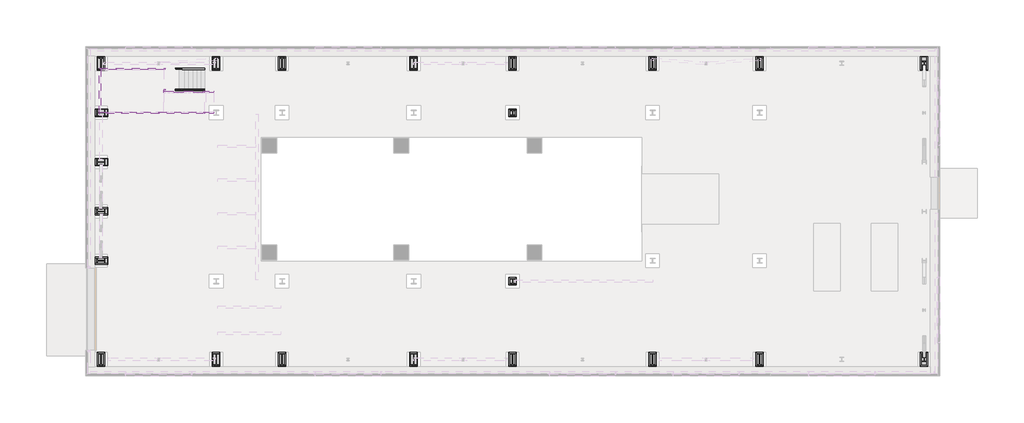
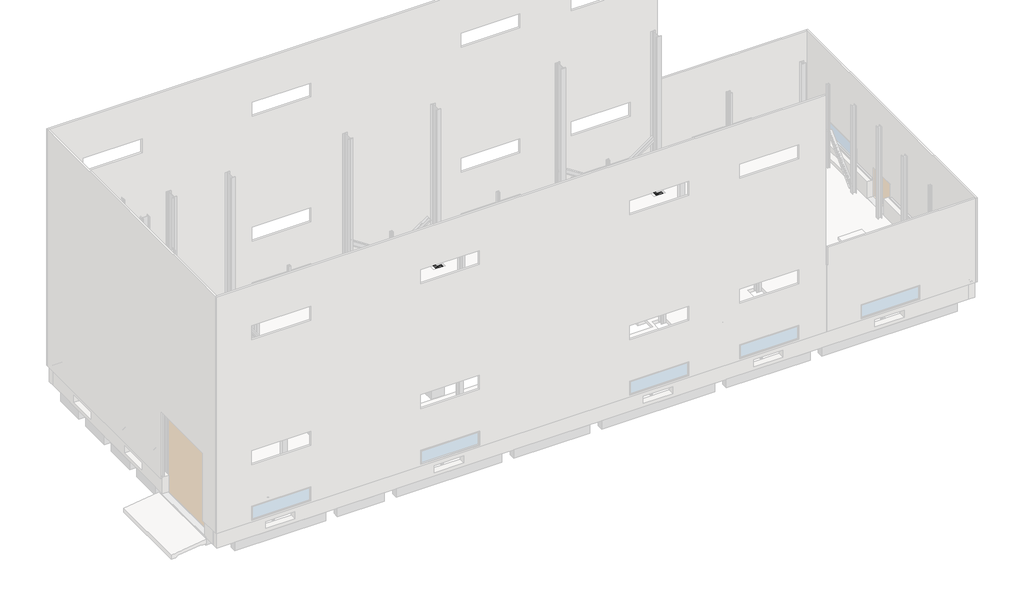
# One storey, part 4 of 4: 23 proxies, 10 members.
# Revit data of these elements (continued)
# Type "그라우트9 : 그라우트"
#   Description = ""
# Type "C-250X90"
#   Keynote = "ㄷ-250×90x9x13"
# Element 1 (IfcBuildingElementProxy, "그라우트 : 그라우트")
#   Phase Created = New Construction
# Element 2 (IfcBuildingElementProxy, "그라우트1 : 그라우트")
#   Phase Created = New Construction
# Element 3 (IfcBuildingElementProxy, "그라우트2 : 그라우트")
#   Phase Created = New Construction
# Element 4 (IfcBuildingElementProxy, "그라우트3 : 그라우트")
#   Phase Created = New Construction
# Element 5 (IfcBuildingElementProxy, "그라우트4 : 그라우트")
#   Phase Created = New Construction
# Element 6 (IfcBuildingElementProxy, "그라우트5 : 그라우트")
#   Phase Created = New Construction
# Element 7 (IfcBuildingElementProxy, "그라우트6 : 그라우트")
#   Phase Created = New Construction
# Element 8 (IfcBuildingElementProxy, "그라우트7 : 그라우트")
#   Phase Created = New Construction
# Element 9 (IfcBuildingElementProxy, "그라우트8 : 그라우트")
#   Phase Created = New Construction
# Element 10 (IfcBuildingElementProxy, "그라우트9 : 그라우트")
#   Phase Created = New Construction
# Element 11 (IfcBuildingElementProxy, "그라우트10 : 그라우트")
#   Phase Created = New Construction
# Element 12 (IfcBuildingElementProxy, "그라우트11 : 그라우트")
#   Phase Created = New Construction
# Element 13 (IfcBuildingElementProxy, "그라우트12 : 그라우트")
#   Phase Created = New Construction
# Element 14 (IfcBuildingElementProxy, "그라우트13 : 그라우트")
#   Phase Created = New Construction
# Element 15 (IfcBuildingElementProxy, "그라우트14 : 그라우트")
#   Phase Created = New Construction
# Element 16 (IfcBuildingElementProxy, "그라우트15 : 그라우트")
#   Phase Created = New Construction
# Element 17 (IfcBuildingElementProxy, "그라우트16 : 그라우트")
#   Phase Created = New Construction
# Element 18 (IfcBuildingElementProxy, "그라우트17 : 그라우트")
#   Phase Created = New Construction
# Element 19 (IfcBuildingElementProxy, "그라우트18 : 그라우트")
#   Phase Created = New Construction
# Element 20 (IfcBuildingElementProxy, "그라우트20 : 그라우트")
#   Phase Created = New Construction
# Element 21 (IfcBuildingElementProxy, "그라우트22 : 그라우트")
#   Phase Created = New Construction
# Element 22 (IfcBuildingElementProxy, "그라우트23 : 그라우트")
#   Phase Created = New Construction
# Element 23 (IfcBuildingElementProxy, "그라우트19 : 그라우트")
#   Phase Created = New Construction
# Elements 24, 25, 26, 27, 28, 29, 30, 31, 32, 33 (IfcMember, "C-250X90")
#   Mark = "ST1"
#   Phase Created = New Construction
#   Materials on its faces: "SM490"
# Materials
#   "SM490": class "Unassigned", colour RGB 84 83 81, transparency 0
# Room at (31078.827, 30248.358) mm, phase "New Construction", upper level "1ST T.O.C", upper offset 2.0000 m, lower offset 0.0000 m
#   Comments = ""
#   Number = "101"
#   Name = "TURBINE HALL"
